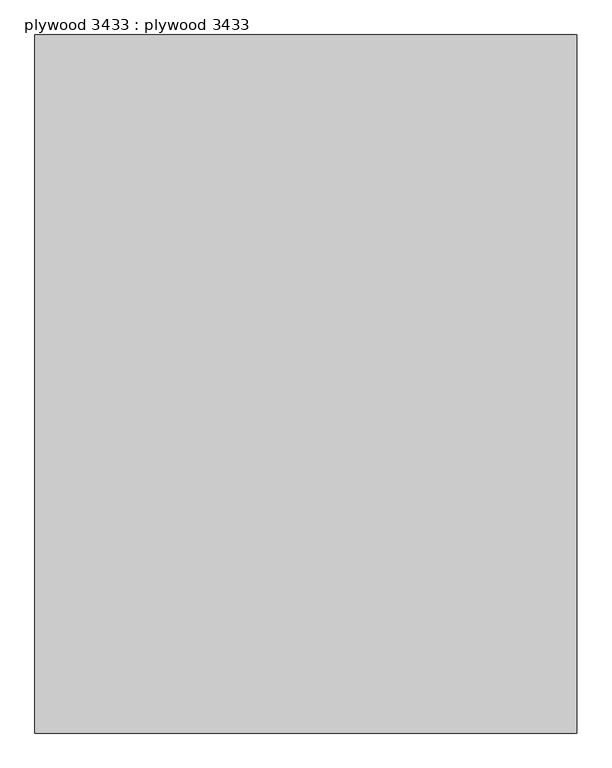
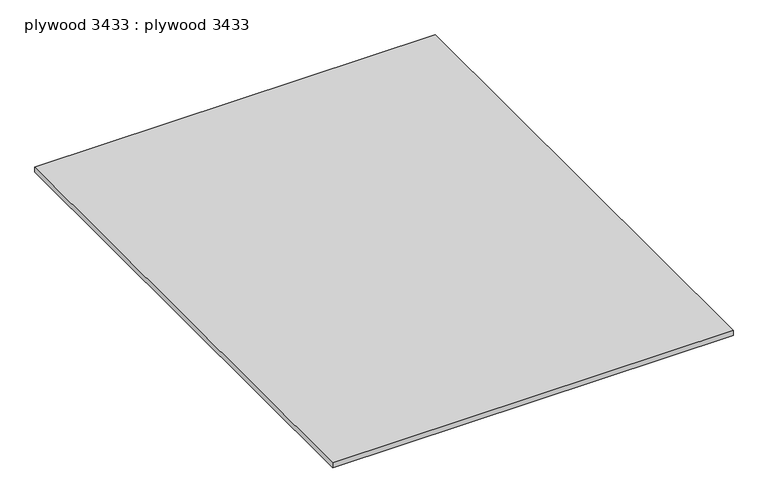
"""IFC4 building model written with IfcOpenShell, lengths in millimetres: proxy geometry, plywood 3433 : plywood 3433."""

from ifc_helpers import new_model, si_unit, frame, origin, place, context, project, spatial, polyline, outline, extrude, source, transform, mapped, element, save


def plywood_3433_plywood_3433_dabd54c6(model_context):
    return source(origin(), model_context, "Body", "SweptSolid", [
        extrude(outline(polyline([(3694.2883192, 7656.2019481), (3694.2883192, 10233.5750834), (5694.2883192, 10233.5750834), (5694.2883192, 7656.2019481), (3694.2883192, 7656.2019481)])), frame((0.0, 0.0, 40112.696), z_axis=(0.0, 0.0, 1.0), x_axis=(1.0, 0.0, 0.0)), (0.0, 0.0, 1.0), 25.4016563),
    ])


if __name__ == "__main__":
    model = new_model("IFC4")
    model_context = context("Model", 3, world=origin())
    ifc_project = project(units=[si_unit("LENGTHUNIT", "METRE", prefix="MILLI")], contexts=[model_context])
    site = spatial("IfcSite", under=ifc_project)
    building = spatial("IfcBuilding", under=site)
    placement = place(None, origin())
    plywood_3433_plywood_3433_shape = plywood_3433_plywood_3433_dabd54c6(model_context)
    element("IfcBuildingElementProxy", 1, Name="plywood 3433 : plywood 3433", ObjectType="plywood 3433 : plywood 3433", at=placement, inside=building, context=model_context, shape_type="MappedRepresentation", body=[
        mapped(plywood_3433_plywood_3433_shape, transform((0.0, 0.0, 0.0), x_axis=(1.0, 0.0, 0.0), y_axis=(0.0, 1.0, 0.0), z_axis=(0.0, 0.0, 1.0))),
    ])
    save(model, "model.ifc")

# Revit data of these elements
# Type "plywood 3433 : plywood 3433"
#   NameOverride = "plywood"
# Element 1 (IfcBuildingElementProxy, "plywood 3433 : plywood 3433")
#   Materials on its faces: "CDX PLYWOOD - SEE STRUCTURAL DWGS"
# Materials
#   "CDX PLYWOOD - SEE STRUCTURAL DWGS": class "Unassigned", colour RGB 177 130 114, transparency 0, Cost = 0
